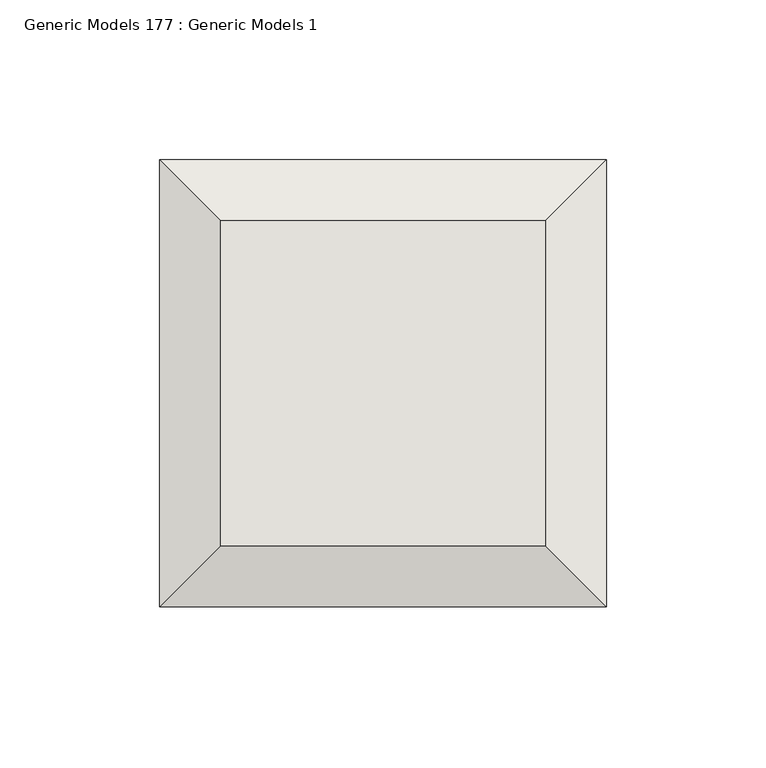
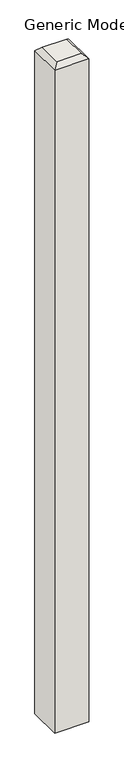
"""IFC4 building model written with IfcOpenShell, lengths in millimetres: wall geometry, Generic Models 177 : Generic Models 1."""

from ifc_helpers import new_model, si_unit, origin, place, context, project, spatial, faceted_brep, source, transform, mapped, element, save


def generic_models_177_generic_models_1_1d143019(model_context):
    return source(origin(), model_context, "Body", "Brep", [
        faceted_brep([(56665.8125, 528.6375, -1066.8), (56526.1125, 528.6375, -1066.8), (56526.1125, 528.6375, 1809.75), (56665.8125, 528.6375, 1809.75), (56665.8125, 388.9375, -1066.8), (56665.8125, 388.9375, 1809.75), (56526.1125, 388.9375, 1809.75), (56526.1125, 388.9375, -1066.8), (56545.1625, 407.9875, 1828.8), (56646.7625, 407.9875, 1828.8), (56646.7625, 509.5875, 1828.8), (56545.1625, 509.5875, 1828.8)], [[[0, 1, 2, 3]], [[4, 5, 6, 7]], [[1, 0, 4, 7]], [[2, 1, 7, 6]], [[8, 9, 10, 11]], [[0, 3, 5, 4]], [[2, 6, 8, 11]], [[5, 3, 10, 9]], [[6, 5, 9, 8]], [[3, 2, 11, 10]]]),
    ])


if __name__ == "__main__":
    model = new_model("IFC4")
    model_context = context("Model", 3, world=origin())
    ifc_project = project(units=[si_unit("LENGTHUNIT", "METRE", prefix="MILLI")], contexts=[model_context])
    site = spatial("IfcSite", under=ifc_project)
    building = spatial("IfcBuilding", under=site)
    placement = place(None, origin())
    generic_models_177_generic_models_1_shape = generic_models_177_generic_models_1_1d143019(model_context)
    element("IfcWall", 1, ObjectType="Generic Models 177 : Generic Models 1", at=placement, inside=building, context=model_context, shape_type="MappedRepresentation", body=[
        mapped(generic_models_177_generic_models_1_shape, transform((0.0, 0.0, 0.0), x_axis=(1.0, 0.0, 0.0), y_axis=(0.0, 1.0, 0.0), z_axis=(0.0, 0.0, 1.0))),
    ])
    save(model, "model.ifc")

# Revit data of these elements
# Element 1 (IfcWall, "Generic Models 177 : Generic Models 1")
#   Materials on its faces: "TREATED 6X6 POST"
# Materials
#   "TREATED 6X6 POST": class "Wood", colour RGB 234 198 147, transparency 0, Description = "Pinus Echinata", Cost = 0
